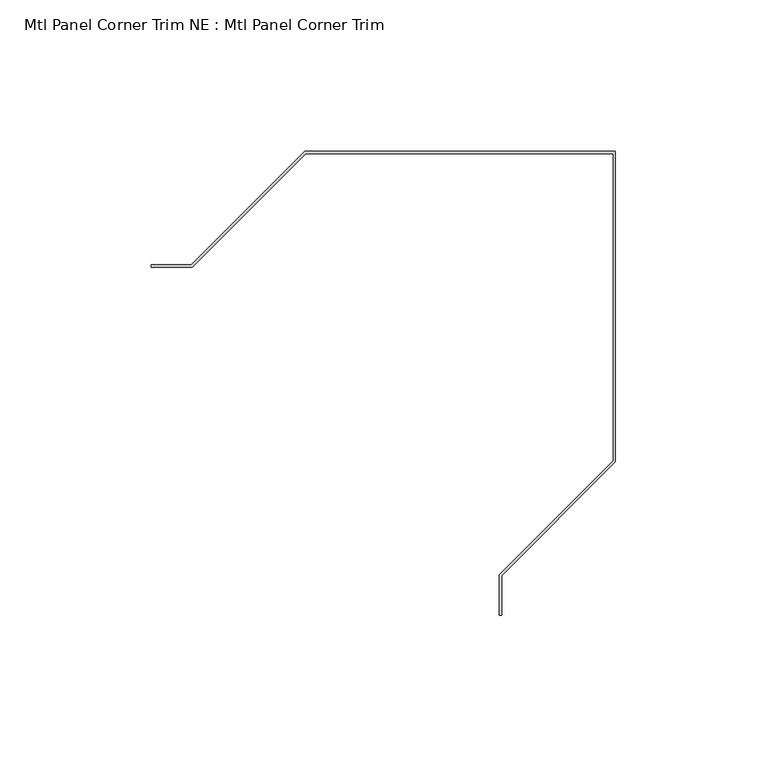
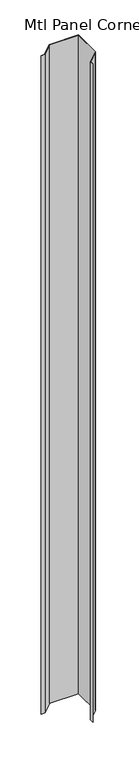
"""IFC4 building model written with IfcOpenShell, lengths in millimetres: proxy geometry, Mtl Panel Corner Trim NE : Mtl Panel Corner Trim."""

from ifc_helpers import new_model, si_unit, frame, origin, place, context, project, spatial, polyline, outline, extrude, source, transform, mapped, element, save


def mtl_panel_corner_trim_ne_mtl_panel_corner_trim_1dc4974f(model_context):
    return source(origin(), model_context, "Body", "SweptSolid", [
        extrude(outline(polyline([(590354.0764739, -531753.7703841), (590354.0764739, -531740.2994038), (590391.6621239, -531702.7137538), (590391.6621239, -531601.1227341), (590290.0711042, -531601.1227341), (590252.5807042, -531638.6131341), (590239.0144739, -531638.6131341), (590239.0144739, -531637.8193841), (590252.2519222, -531637.8193841), (590289.7423222, -531600.3289841), (590392.4558739, -531600.3289841), (590392.4558739, -531703.0425358), (590354.8638739, -531740.6345358), (590354.8638739, -531753.7703841), (590354.0764739, -531753.7703841)])), frame((0.0, 0.0, 6.35), z_axis=(0.0, 0.0, 1.0), x_axis=(1.0, 0.0, 0.0)), (0.0, 0.0, 1.0), 2432.05),
    ])


if __name__ == "__main__":
    model = new_model("IFC4")
    model_context = context("Model", 3, world=origin())
    ifc_project = project(units=[si_unit("LENGTHUNIT", "METRE", prefix="MILLI")], contexts=[model_context])
    site = spatial("IfcSite", under=ifc_project)
    building = spatial("IfcBuilding", under=site)
    placement = place(None, origin())
    mtl_panel_corner_trim_ne_mtl_panel_corner_trim_shape = mtl_panel_corner_trim_ne_mtl_panel_corner_trim_1dc4974f(model_context)
    element("IfcBuildingElementProxy", 1, Name="Mtl Panel Corner Trim NE : Mtl Panel Corner Trim", ObjectType="Mtl Panel Corner Trim NE : Mtl Panel Corner Trim", at=placement, inside=building, context=model_context, shape_type="MappedRepresentation", body=[
        mapped(mtl_panel_corner_trim_ne_mtl_panel_corner_trim_shape, transform((0.0, 0.0, 0.0), x_axis=(1.0, 0.0, 0.0), y_axis=(0.0, 1.0, 0.0), z_axis=(0.0, 0.0, 1.0))),
    ])
    save(model, "model.ifc")

# Revit data of these elements
# Element 1 (IfcBuildingElementProxy, "Mtl Panel Corner Trim NE : Mtl Panel Corner Trim")
#   Materials on its faces: "CORNER TRIM BY MTL PANEL MFR."
# Materials
#   "CORNER TRIM BY MTL PANEL MFR.": class "Generic", colour RGB 239 242 240, transparency 0, Cost = 0
